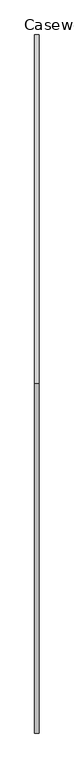
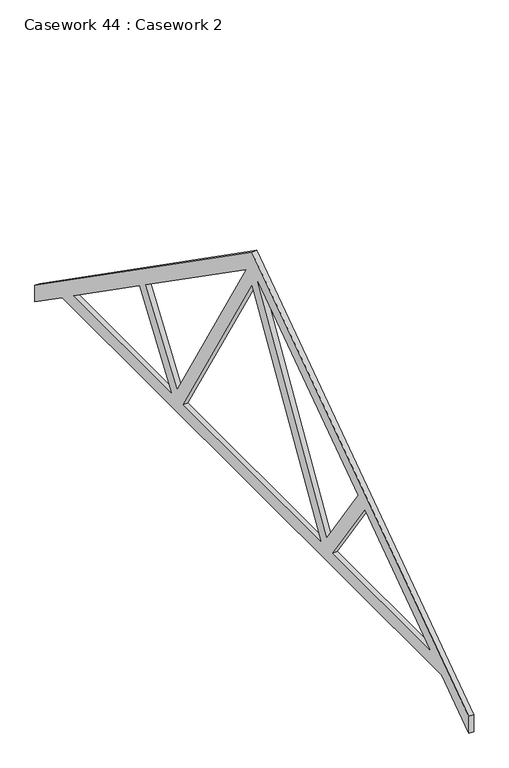
"""IFC4 building model written with IfcOpenShell, lengths in millimetres: furniture geometry, Casework 44 : Casework 2."""

from ifc_helpers import new_model, si_unit, frame, origin, place, context, project, spatial, polyline, outline, extrude, source, transform, mapped, element, save


def casework_44_casework_2_18aa97ba(model_context):
    return source(origin(), model_context, "Body", "SweptSolid", [
        extrude(outline(polyline([(6583.1149316, 5250.0), (-277.3850684, 5250.0), (-767.3850684, 4906.8983063), (-767.3850684, 5090.0144946), (3152.8649316, 7835.0030963), (7073.1149316, 5090.0144946), (7073.1149316, 4906.8983063), (6583.1149316, 5250.0)]), holes=[polyline([(4612.3149663, 5400.0), (6368.8927306, 5400.0), (5190.2113591, 6225.3215815), (4612.3149663, 5400.0)]), polyline([(4394.2037684, 5400.0), (3152.8649316, 7465.9347567), (1911.5260948, 5400.0), (4394.2037684, 5400.0)]), polyline([(4504.5438357, 5507.6038939), (5067.3385525, 6311.3580469), (3262.0771677, 7575.415677), (4504.5438357, 5507.6038939)]), polyline([(1693.4148969, 5400.0), (1115.5185041, 6225.3215815), (-63.1628674, 5400.0), (1693.4148969, 5400.0)]), polyline([(1801.1860276, 5507.6038939), (3043.6526956, 7575.415677), (1238.3913108, 6311.3580469), (1801.1860276, 5507.6038939)])]), frame((-9221.5247381, 0.0, 0.0), z_axis=(1.0, 0.0, 0.0), x_axis=(0.0, 1.0, 0.0)), (0.0, 0.0, 1.0), 49.6351915),
    ])


if __name__ == "__main__":
    model = new_model("IFC4")
    model_context = context("Model", 3, world=origin())
    ifc_project = project(units=[si_unit("LENGTHUNIT", "METRE", prefix="MILLI")], contexts=[model_context])
    site = spatial("IfcSite", under=ifc_project)
    building = spatial("IfcBuilding", under=site)
    placement = place(None, origin())
    casework_44_casework_2_shape = casework_44_casework_2_18aa97ba(model_context)
    element("IfcFurniture", 1, ObjectType="Casework 44 : Casework 2", at=placement, inside=building, context=model_context, shape_type="MappedRepresentation", body=[
        mapped(casework_44_casework_2_shape, transform((0.0, 0.0, 0.0), x_axis=(1.0, 0.0, 0.0), y_axis=(0.0, 1.0, 0.0), z_axis=(0.0, 0.0, 1.0))),
    ])
    save(model, "model.ifc")

# Revit data of these elements
# Element 1 (IfcFurniture, "Casework 44 : Casework 2")
#   Materials on its faces: "Softwood, Lumber"
# Materials
#   "Softwood, Lumber": class "Wood", colour RGB 205 156 65, transparency 0, Description = "Pinus Echinata", Cost = 0
